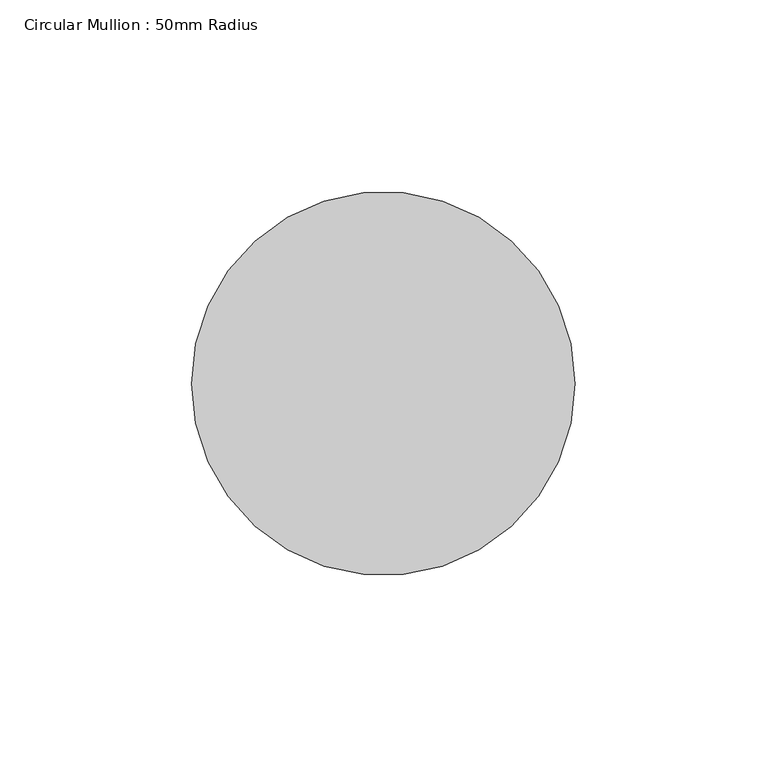
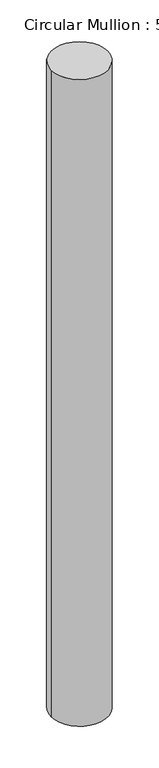
"""IFC4 building model written with IfcOpenShell, lengths in millimetres: member geometry, Circular Mullion : 50mm Radius."""

from ifc_helpers import new_model, si_unit, point, frame, origin, origin_2d, place, context, project, spatial, circle_curve, trimmed, segment, composite_curve, outline, extrude, source, transform, mapped, element, save


def circular_mullion_50mm_radius_f224f08a(model_context):
    return source(origin(), model_context, "Body", "SweptSolid", [
        extrude(outline(composite_curve([segment(trimmed(circle_curve(origin_2d(), 50.0), [point((50.0, 0.0))], [point((-50.0, 0.0))], False, "CARTESIAN"), True, "CONTINUOUS"), segment(trimmed(circle_curve(origin_2d(), 50.0), [point((-50.0, 0.0))], [point((50.0, 0.0))], False, "CARTESIAN"), True, "CONTINUOUS")], self_intersect=False)), frame((0.0, 0.0, -1202.7134938), z_axis=(0.0, 0.0, 1.0), x_axis=(1.0, 0.0, 0.0)), (0.0, 0.0, 1.0), 1202.7134938),
    ])


if __name__ == "__main__":
    model = new_model("IFC4")
    model_context = context("Model", 3, world=origin())
    ifc_project = project(units=[si_unit("LENGTHUNIT", "METRE", prefix="MILLI")], contexts=[model_context])
    site = spatial("IfcSite", under=ifc_project)
    building = spatial("IfcBuilding", under=site)
    placement = place(None, origin())
    circular_mullion_50mm_radius_shape = circular_mullion_50mm_radius_f224f08a(model_context)
    element("IfcMember", 1, ObjectType="Circular Mullion : 50mm Radius", at=placement, inside=building, context=model_context, shape_type="MappedRepresentation", body=[
        mapped(circular_mullion_50mm_radius_shape, transform((0.0, 0.0, 0.0), x_axis=(1.0, 0.0, 0.0), y_axis=(0.0, 1.0, 0.0), z_axis=(0.0, 0.0, 1.0))),
    ])
    save(model, "model.ifc")

# Revit data of these elements
# Type "Circular Mullion : 50mm Radius"
#   built-in parameter 1007350 = 0.164042 (stored number, unit not read)
# Element 1 (IfcMember, "Circular Mullion : 50mm Radius")
#   Materials on its faces: "Aluminium"
# Materials
#   "Aluminium": class "Metal", colour RGB 247 247 247, transparency 0, Description = "Aluminium 6061", Cost = 0
